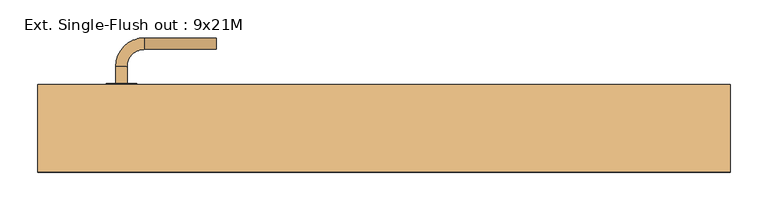
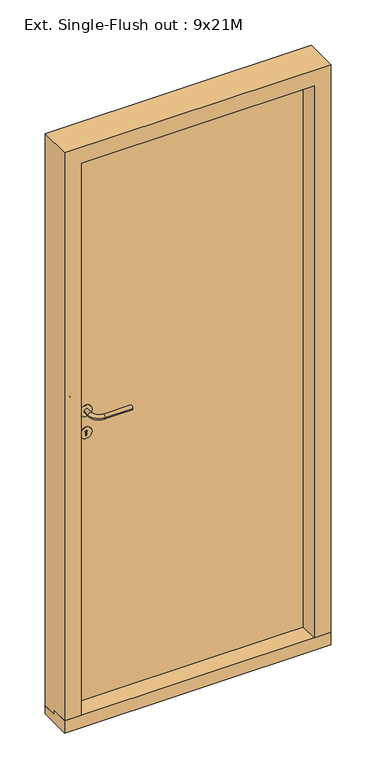
"""IFC4 building model written with IfcOpenShell, lengths in millimetres: door geometry, Ext. Single-Flush out : 9x21M."""

from ifc_helpers import new_model, si_unit, point, frame, frame_2d, origin, place, context, project, spatial, polyline, circle_curve, ellipse_curve, trimmed, segment, composite_curve, outline, extrude, faceted_brep, source, transform, mapped, element, save
from ifc_brep_helpers import plane_surface, cylinder_surface, revolved_surface, advanced_brep


def ext_single_flush_out_9x21m_755ac03d(model_context):
    return source(origin(), model_context, "Body", "SolidModel", [
        extrude(outline(composite_curve([segment(trimmed(circle_curve(frame_2d((1090.0, -346.0)), 20.0), [point((1070.0, -346.0))], [point((1110.0, -346.0))], False, "CARTESIAN"), True, "CONTINUOUS"), segment(trimmed(circle_curve(frame_2d((1090.0, -346.0)), 20.0), [point((1110.0, -346.0))], [point((1070.0, -346.0))], False, "CARTESIAN"), True, "CONTINUOUS")], self_intersect=False)), frame((0.0, 184.0, 0.0), z_axis=(0.0, 1.0, 0.0), x_axis=(0.0, 0.0, 1.0)), (0.0, 0.0, 1.0), 2.0),
        advanced_brep(
        [(-353.5, 186.0, 1090.0), (-338.5, 186.0, 1090.0), (-353.5, 208.5, 1090.0), (-338.5, 208.5, 1090.0), (-316.0, 231.0, 1090.0), (-316.0, 246.0, 1090.0), (-221.0, 246.0, 1090.0), (-221.0, 231.0, 1090.0)],
        [
            (0, 1, circle_curve(frame((-346.0, 186.0, 1090.0), z_axis=(0.0, -1.0, 0.0), x_axis=(1.0, 0.0, 0.0)), 7.5)),
            (1, 0, circle_curve(frame((-346.0, 186.0, 1090.0), z_axis=(0.0, -1.0, 0.0), x_axis=(1.0, 0.0, 0.0)), 7.5)),
            (0, 2),
            (2, 3, circle_curve(frame((-346.0, 208.5, 1090.0), z_axis=(0.0, -1.0, 0.0), x_axis=(1.0, 0.0, 0.0)), 7.5)),
            (3, 1),
            (3, 2, circle_curve(frame((-346.0, 208.5, 1090.0), z_axis=(0.0, -1.0, 0.0), x_axis=(1.0, 0.0, 0.0)), 7.5)),
            (4, 3, circle_curve(frame((-316.0, 208.5, 1090.0), z_axis=(0.0, 0.0, 1.0), x_axis=(-1.0, 0.0, 0.0)), 22.5)),
            (2, 5, circle_curve(frame((-316.0, 208.5, 1090.0), z_axis=(0.0, 0.0, -1.0), x_axis=(-1.0, 0.0, 0.0)), 37.5)),
            (5, 4, circle_curve(frame((-316.0, 238.5, 1090.0), z_axis=(-1.0, 0.0, 0.0), x_axis=(0.0, -1.0, 0.0)), 7.5)),
            (4, 5, circle_curve(frame((-316.0, 238.5, 1090.0), z_axis=(-1.0, 0.0, 0.0), x_axis=(0.0, -1.0, 0.0)), 7.5)),
            (5, 6),
            (6, 7, circle_curve(frame((-221.0, 238.5, 1090.0), z_axis=(-1.0, 0.0, 0.0), x_axis=(0.0, -1.0, 0.0)), 7.5)),
            (7, 4),
            (7, 6, circle_curve(frame((-221.0, 238.5, 1090.0), z_axis=(-1.0, 0.0, 0.0), x_axis=(0.0, -1.0, 0.0)), 7.5)),
        ],
        [
            plane_surface(frame((-346.0, 186.0, 1090.0), z_axis=(0.0, -1.0, 0.0), x_axis=(0.0, 0.0, -1.0))),
            cylinder_surface(frame((-346.0, 186.0, 1090.0), z_axis=(0.0, -1.0, 0.0), x_axis=(1.0, 0.0, 0.0)), 7.5),
            revolved_surface(trimmed(ellipse_curve(frame((-346.0, 208.5, 1090.0), z_axis=(0.0, -1.0, 0.0), x_axis=(1.0, 0.0, 0.0)), 7.5, 7.5), [point((-353.5, 208.5, 1090.0))], [point((-338.5, 208.5, 1090.0))], True, "CARTESIAN"), (-316.0, 208.5, 1090.0), (0.0, 0.0, -1.0)),
            revolved_surface(trimmed(ellipse_curve(frame((-346.0, 208.5, 1090.0), z_axis=(0.0, -1.0, 0.0), x_axis=(1.0, 0.0, 0.0)), 7.5, 7.5), [point((-338.5, 208.5, 1090.0))], [point((-353.5, 208.5, 1090.0))], True, "CARTESIAN"), (-316.0, 208.5, 1090.0), (0.0, 0.0, -1.0)),
            cylinder_surface(frame((-316.0, 238.5, 1090.0), z_axis=(-1.0, 0.0, 0.0), x_axis=(0.0, -1.0, 0.0)), 7.5),
            plane_surface(frame((-221.0, 238.5, 1090.0), z_axis=(1.0, 0.0, 0.0), x_axis=(0.0, 0.0, -1.0))),
        ],
        [
            (0, [[1, 2]]),
            (1, [[-1, 3, 4, 5]]),
            (1, [[-2, -5, 6, -3]]),
            (2, [[7, -4, 8, 9]]),
            (3, [[-8, -6, -7, 10]]),
            (4, [[-9, 11, 12, 13]]),
            (4, [[-10, -13, 14, -11]]),
            (5, [[-14, -12]]),
        ],
    ),
        extrude(outline(composite_curve([segment(trimmed(circle_curve(frame_2d((1010.0, -346.0)), 20.0), [point((990.0, -346.0))], [point((1030.0, -346.0))], False, "CARTESIAN"), True, "CONTINUOUS"), segment(trimmed(circle_curve(frame_2d((1010.0, -346.0)), 20.0), [point((1030.0, -346.0))], [point((990.0, -346.0))], False, "CARTESIAN"), True, "CONTINUOUS")], self_intersect=False), holes=[composite_curve([segment(trimmed(circle_curve(frame_2d((1015.0, -346.0)), 3.0), [point((1012.4019238, -347.5))], [point((1012.4019238, -344.5))], True, "CARTESIAN"), True, "CONTINUOUS"), segment(polyline([(1012.4019238, -344.5), (1000.0, -344.5), (1000.0, -347.5), (1012.4019238, -347.5)]), True, "CONTINUOUS")], self_intersect=False)]), frame((0.0, 184.0, 0.0), z_axis=(0.0, 1.0, 0.0), x_axis=(0.0, 0.0, 1.0)), (0.0, 0.0, 1.0), 2.0),
        extrude(outline(composite_curve([segment(trimmed(circle_curve(frame_2d((1090.0, -346.0)), 20.0), [point((1070.0, -346.0))], [point((1110.0, -346.0))], False, "CARTESIAN"), True, "CONTINUOUS"), segment(trimmed(circle_curve(frame_2d((1090.0, -346.0)), 20.0), [point((1110.0, -346.0))], [point((1070.0, -346.0))], False, "CARTESIAN"), True, "CONTINUOUS")], self_intersect=False)), frame((0.0, 132.0, 0.0), z_axis=(0.0, 1.0, 0.0), x_axis=(0.0, 0.0, 1.0)), (0.0, 0.0, 1.0), 2.0),
        advanced_brep(
        [(-353.5, 132.0, 1090.0), (-338.5, 132.0, 1090.0), (-338.5, 109.5, 1090.0), (-353.5, 109.5, 1090.0), (-316.0, 87.0, 1090.0), (-316.0, 72.0, 1090.0), (-221.0, 87.0, 1090.0), (-221.0, 72.0, 1090.0)],
        [
            (0, 1, circle_curve(frame((-346.0, 132.0, 1090.0), z_axis=(0.0, 1.0, 0.0), x_axis=(1.0, 0.0, 0.0)), 7.5)),
            (1, 0, circle_curve(frame((-346.0, 132.0, 1090.0), z_axis=(0.0, 1.0, 0.0), x_axis=(1.0, 0.0, 0.0)), 7.5)),
            (1, 2),
            (2, 3, circle_curve(frame((-346.0, 109.5, 1090.0), z_axis=(0.0, 1.0, 0.0), x_axis=(1.0, 0.0, 0.0)), 7.5)),
            (3, 0),
            (3, 2, circle_curve(frame((-346.0, 109.5, 1090.0), z_axis=(0.0, 1.0, 0.0), x_axis=(1.0, 0.0, 0.0)), 7.5)),
            (4, 5, circle_curve(frame((-316.0, 79.5, 1090.0), z_axis=(-1.0, 0.0, 0.0), x_axis=(0.0, 1.0, 0.0)), 7.5)),
            (5, 3, circle_curve(frame((-316.0, 109.5, 1090.0), z_axis=(0.0, 0.0, -1.0), x_axis=(-1.0, 0.0, 0.0)), 37.5)),
            (2, 4, circle_curve(frame((-316.0, 109.5, 1090.0), z_axis=(0.0, 0.0, 1.0), x_axis=(-1.0, 0.0, 0.0)), 22.5)),
            (5, 4, circle_curve(frame((-316.0, 79.5, 1090.0), z_axis=(-1.0, 0.0, 0.0), x_axis=(0.0, 1.0, 0.0)), 7.5)),
            (4, 6),
            (6, 7, circle_curve(frame((-221.0, 79.5, 1090.0), z_axis=(-1.0, 0.0, 0.0), x_axis=(0.0, 1.0, 0.0)), 7.5)),
            (7, 5),
            (7, 6, circle_curve(frame((-221.0, 79.5, 1090.0), z_axis=(-1.0, 0.0, 0.0), x_axis=(0.0, 1.0, 0.0)), 7.5)),
        ],
        [
            plane_surface(frame((-346.0, 132.0, 1090.0), z_axis=(0.0, 1.0, 0.0), x_axis=(0.0, 0.0, -1.0))),
            cylinder_surface(frame((-346.0, 132.0, 1090.0), z_axis=(0.0, 1.0, 0.0), x_axis=(1.0, 0.0, 0.0)), 7.5),
            revolved_surface(trimmed(ellipse_curve(frame((-346.0, 109.5, 1090.0), z_axis=(0.0, -1.0, 0.0), x_axis=(1.0, 0.0, 0.0)), 7.5, 7.5), [point((-353.5, 109.5, 1090.0))], [point((-338.5, 109.5, 1090.0))], True, "CARTESIAN"), (-316.0, 109.5, 1090.0), (0.0, 0.0, -1.0)),
            revolved_surface(trimmed(ellipse_curve(frame((-346.0, 109.5, 1090.0), z_axis=(0.0, -1.0, 0.0), x_axis=(1.0, 0.0, 0.0)), 7.5, 7.5), [point((-338.5, 109.5, 1090.0))], [point((-353.5, 109.5, 1090.0))], True, "CARTESIAN"), (-316.0, 109.5, 1090.0), (0.0, 0.0, -1.0)),
            cylinder_surface(frame((-316.0, 79.5, 1090.0), z_axis=(-1.0, 0.0, 0.0), x_axis=(0.0, 1.0, 0.0)), 7.5),
            plane_surface(frame((-221.0, 79.5, 1090.0), z_axis=(1.0, 0.0, 0.0), x_axis=(0.0, 0.0, -1.0))),
        ],
        [
            (0, [[1, 2]]),
            (1, [[3, 4, 5, -2]]),
            (1, [[-5, 6, -3, -1]]),
            (2, [[7, 8, -4, 9]]),
            (3, [[10, -9, -6, -8]]),
            (4, [[11, 12, 13, -7]]),
            (4, [[-13, 14, -11, -10]]),
            (5, [[-12, -14]]),
        ],
    ),
        extrude(outline(composite_curve([segment(trimmed(circle_curve(frame_2d((1010.0, -346.0)), 20.0), [point((990.0, -346.0))], [point((1030.0, -346.0))], False, "CARTESIAN"), True, "CONTINUOUS"), segment(trimmed(circle_curve(frame_2d((1010.0, -346.0)), 20.0), [point((1030.0, -346.0))], [point((990.0, -346.0))], False, "CARTESIAN"), True, "CONTINUOUS")], self_intersect=False), holes=[composite_curve([segment(trimmed(circle_curve(frame_2d((1015.0, -346.0)), 3.0), [point((1012.4019238, -347.5))], [point((1012.4019238, -344.5))], True, "CARTESIAN"), True, "CONTINUOUS"), segment(polyline([(1012.4019238, -344.5), (1000.0, -344.5), (1000.0, -347.5), (1012.4019238, -347.5)]), True, "CONTINUOUS")], self_intersect=False)]), frame((0.0, 132.0, 0.0), z_axis=(0.0, 1.0, 0.0), x_axis=(0.0, 0.0, 1.0)), (0.0, 0.0, 1.0), 2.0),
        extrude(outline(polyline([(-414.0, 184.0), (414.0, 184.0), (414.0, 134.0), (-414.0, 134.0), (-414.0, 184.0)])), frame((0.0, 0.0, 30.0), z_axis=(0.0, 0.0, 1.0), x_axis=(1.0, 0.0, 0.0)), (0.0, 0.0, 1.0), 2028.0),
        faceted_brep([(414.0, 184.0, 2058.0), (-414.0, 184.0, 2058.0), (-414.0, 184.0, 30.0), (-456.0, 184.0, 30.0), (-456.0, 184.0, 2100.0), (456.0, 184.0, 2100.0), (456.0, 184.0, 30.0), (414.0, 184.0, 30.0), (-414.0, 134.0, 2058.0), (-414.0, 134.0, 45.0), (-414.0, 134.0, 30.0), (456.0, 134.0, 30.0), (414.0, 134.0, 30.0), (-456.0, 134.0, 30.0), (-456.0, 69.0, 2100.0), (-456.0, 134.0, 45.0), (-456.0, 69.0, 45.0), (456.0, 69.0, 2100.0), (456.0, 69.0, 45.0), (456.0, 134.0, 45.0), (414.0, 134.0, 2058.0), (414.0, 134.0, 45.0), (-399.0, 69.0, 45.0), (-399.0, 69.0, 2043.0), (399.0, 69.0, 2043.0), (399.0, 69.0, 45.0), (399.0, 134.0, 45.0), (-399.0, 134.0, 45.0), (-399.0, 134.0, 2043.0), (399.0, 134.0, 2043.0)], [[[0, 1, 2, 3, 4, 5, 6, 7]], [[1, 8, 9, 10, 2]], [[11, 12, 7, 6]], [[10, 13, 3, 2]], [[14, 4, 3, 13, 15, 16]], [[5, 17, 18, 19, 11, 6]], [[20, 0, 7, 12, 21]], [[17, 14, 16, 22, 23, 24, 25, 18]], [[21, 19, 18, 25, 26]], [[15, 9, 27, 22, 16]], [[19, 21, 12, 11]], [[9, 15, 13, 10]], [[28, 23, 22, 27]], [[24, 29, 26, 25]], [[29, 28, 27, 9, 8, 20, 21, 26]], [[5, 4, 14, 17]], [[24, 23, 28, 29]], [[1, 0, 20, 8]]]),
        extrude(outline(polyline([(184.0, 30.0), (184.0, 0.0), (69.0, 0.0), (69.0, 45.0), (134.0, 45.0), (134.0, 30.0), (184.0, 30.0)])), frame((-456.0, 0.0, 0.0), z_axis=(1.0, 0.0, 0.0), x_axis=(0.0, 1.0, 0.0)), (0.0, 0.0, 1.0), 912.0),
    ])


if __name__ == "__main__":
    model = new_model("IFC4")
    model_context = context("Model", 3, world=origin())
    ifc_project = project(units=[si_unit("LENGTHUNIT", "METRE", prefix="MILLI")], contexts=[model_context])
    site = spatial("IfcSite", under=ifc_project)
    building = spatial("IfcBuilding", under=site)
    placement = place(None, origin())
    ext_single_flush_out_9x21m_shape = ext_single_flush_out_9x21m_755ac03d(model_context)
    element("IfcDoor", 1, ObjectType="Ext. Single-Flush out : 9x21M", at=placement, inside=building, context=model_context, shape_type="MappedRepresentation", body=[
        mapped(ext_single_flush_out_9x21m_shape, transform((0.0, 0.0, 0.0), x_axis=(1.0, 0.0, 0.0), y_axis=(0.0, 1.0, 0.0), z_axis=(0.0, 0.0, 1.0))),
    ])
    save(model, "model.ifc")

# Revit data of these elements
# Type "Ext. Single-Flush out : 9x21M"
#   Type Mark = "63"
#   Sound Rating = ""
#   Opening Side [instance default] = "out"
#   Hinge Side [instance default] = ""
#   Creator Organization [instance default] = "© Danish Educational Content"
#   Creator Name [instance default] = "© Erik Falck Jørgensen"
#   Creator Build [instance default] = "2017.0301.0"
#   Analytic Construction = "<None>"
#   length#6 = -50 mm
#   length#4 = 120 mm
#   length#5 = 912 mm
#   length#3 = 30 mm
#   length#2 = 57 mm
#   length#1 = 0 mm
#   Thickness = 50 mm
#   Seal Width = 12 mm
#   Rough Width = 912 mm
#   Rough Height = 2100 mm
#   Rebate Depth = 50 mm
#   Rabbet Width = 15 mm
#   Rabbet Depth = 50 mm
#   Height = 2088 mm
#   Width = 888 mm
#   Handle From Side = 110 mm
#   Handle From Bottom = 1090 mm
#   Exterior Direction [instance default] = 0.00°
#   Case Depth = 115 mm
#   Case Width = 45 mm
#   Threshold = yes
#   Sealing = no
#   Hinging = yes
#   Wall Closure = 1
#   Function = 1
#   Panel = none
#   Handle Finish = none
#   Handle = element 632149
#   Case/Transom = none
#   Assembly Code = ""
# Element 1 (IfcDoor, "Ext. Single-Flush out : 9x21M")
#   Materials on its faces: "Stainless Steel, Polished", "Default Frame/Mullion (Interior/Exterior)", "Default Door Panel (Exterior/Interior)"
# Materials
#   "Stainless Steel, Polished": class "Metal", colour RGB 180 180 180, transparency 0, Description = "Rustfri stål, poleret", Cost = 0
#   "Default Frame/Mullion (Interior/Exterior)": class "Generic", colour RGB 205 205 205, transparency 0, Description = "Udefineret karm/ramme materiale", Cost = 0
#   "Default Door Panel (Exterior/Interior)": class "Generic", colour RGB 205 205 205, transparency 0, Description = "Udefineret dørplade materiale", Cost = 0
